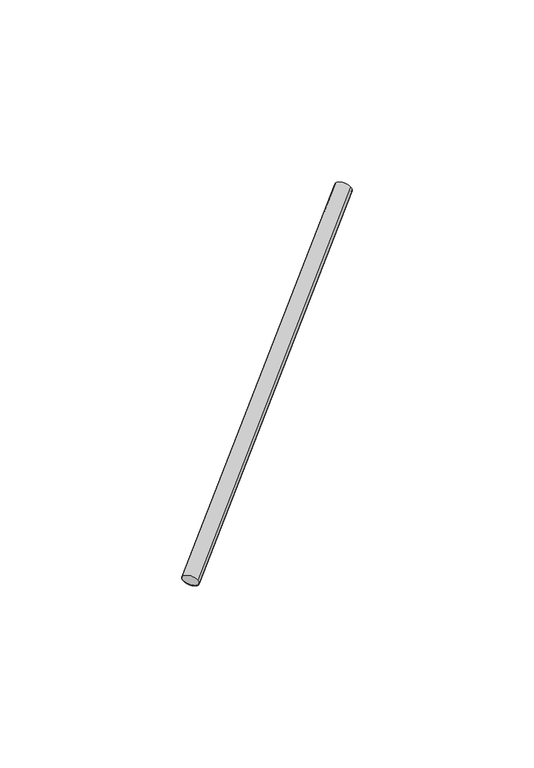
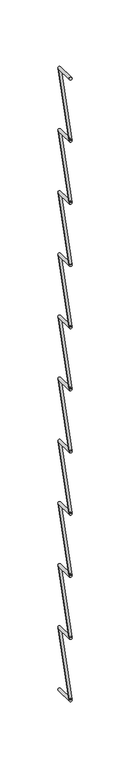
"""IFC4 building model written with IfcOpenShell, lengths in millimetres: proxy geometry, Pre-fab. (Vigota 7 - Pano 3)."""

from ifc_helpers import new_model, si_unit, point, frame, origin, origin_2d, place, context, project, spatial, circle_curve, trimmed, segment, composite_curve, outline, extrude, source, transform, mapped, element, save


def structural_framing_6d4e4e1a(model_context):
    return source(origin(), model_context, "Body", "SweptSolid", [
        extrude(outline(composite_curve([segment(trimmed(circle_curve(origin_2d(), 2.5), [point((2.5, 0.0))], [point((-2.5, 0.0))], False, "CARTESIAN"), True, "CONTINUOUS"), segment(trimmed(circle_curve(origin_2d(), 2.5), [point((-2.5, 0.0))], [point((2.5, 0.0))], False, "CARTESIAN"), True, "CONTINUOUS")], self_intersect=False)), frame((-42.0, 108.0, 1769.500535), z_axis=(-0.3218603428886276, -0.8276408817707567, 0.4598004898837537), x_axis=(0.8192319205108605, 3.936835275445103e-11, 0.5734623443750141)), (0.0, 0.0, 1.0), 130.491379),
        extrude(outline(composite_curve([segment(trimmed(circle_curve(origin_2d(), 2.5), [point((2.5, 0.0))], [point((-2.5, 0.0))], False, "CARTESIAN"), True, "CONTINUOUS"), segment(trimmed(circle_curve(origin_2d(), 2.5), [point((-2.5, 0.0))], [point((2.5, 0.0))], False, "CARTESIAN"), True, "CONTINUOUS")], self_intersect=False)), frame((-84.0, 0.0, 1829.500535), z_axis=(0.3218603428886276, 0.8276408817707567, 0.4598004898837537), x_axis=(0.8192319205108605, 3.936835275445103e-11, -0.5734623443750141)), (0.0, 0.0, 1.0), 130.491379),
        extrude(outline(composite_curve([segment(trimmed(circle_curve(origin_2d(), 2.5), [point((2.5, 0.0))], [point((-2.5, 0.0))], False, "CARTESIAN"), True, "CONTINUOUS"), segment(trimmed(circle_curve(origin_2d(), 2.5), [point((-2.5, 0.0))], [point((2.5, 0.0))], False, "CARTESIAN"), True, "CONTINUOUS")], self_intersect=False)), frame((-42.0, 108.0, 1889.500535), z_axis=(-0.3218603428886276, -0.8276408817707567, 0.4598004898837537), x_axis=(0.8192319205108605, 3.936835275445103e-11, 0.5734623443750141)), (0.0, 0.0, 1.0), 130.491379),
        extrude(outline(composite_curve([segment(trimmed(circle_curve(origin_2d(), 2.5), [point((2.5, 0.0))], [point((-2.5, 0.0))], False, "CARTESIAN"), True, "CONTINUOUS"), segment(trimmed(circle_curve(origin_2d(), 2.5), [point((-2.5, 0.0))], [point((2.5, 0.0))], False, "CARTESIAN"), True, "CONTINUOUS")], self_intersect=False)), frame((-84.0, 0.0, 1949.500535), z_axis=(0.3218603428886276, 0.8276408817707567, 0.4598004898837537), x_axis=(0.8192319205108605, 3.936835275445103e-11, -0.5734623443750141)), (0.0, 0.0, 1.0), 130.491379),
        extrude(outline(composite_curve([segment(trimmed(circle_curve(origin_2d(), 2.5), [point((2.5, 0.0))], [point((-2.5, 0.0))], False, "CARTESIAN"), True, "CONTINUOUS"), segment(trimmed(circle_curve(origin_2d(), 2.5), [point((-2.5, 0.0))], [point((2.5, 0.0))], False, "CARTESIAN"), True, "CONTINUOUS")], self_intersect=False)), frame((-42.0, 108.0, 2009.500535), z_axis=(-0.3218603428886276, -0.8276408817707567, 0.4598004898837537), x_axis=(0.8192319205108605, 3.936835275445103e-11, 0.5734623443750141)), (0.0, 0.0, 1.0), 130.491379),
        extrude(outline(composite_curve([segment(trimmed(circle_curve(origin_2d(), 2.5), [point((2.5, 0.0))], [point((-2.5, 0.0))], False, "CARTESIAN"), True, "CONTINUOUS"), segment(trimmed(circle_curve(origin_2d(), 2.5), [point((-2.5, 0.0))], [point((2.5, 0.0))], False, "CARTESIAN"), True, "CONTINUOUS")], self_intersect=False)), frame((-84.0, 0.0, 2069.500535), z_axis=(0.3218603428886276, 0.8276408817707567, 0.4598004898837537), x_axis=(0.8192319205108605, 3.936835275445103e-11, -0.5734623443750141)), (0.0, 0.0, 1.0), 130.491379),
        extrude(outline(composite_curve([segment(trimmed(circle_curve(origin_2d(), 2.5), [point((2.5, 0.0))], [point((-2.5, 0.0))], False, "CARTESIAN"), True, "CONTINUOUS"), segment(trimmed(circle_curve(origin_2d(), 2.5), [point((-2.5, 0.0))], [point((2.5, 0.0))], False, "CARTESIAN"), True, "CONTINUOUS")], self_intersect=False)), frame((-42.0, 108.0, 2129.500535), z_axis=(-0.3218603428886276, -0.8276408817707567, 0.4598004898837537), x_axis=(0.8192319205108605, 3.936835275445103e-11, 0.5734623443750141)), (0.0, 0.0, 1.0), 130.491379),
        extrude(outline(composite_curve([segment(trimmed(circle_curve(origin_2d(), 2.5), [point((2.5, 0.0))], [point((-2.5, 0.0))], False, "CARTESIAN"), True, "CONTINUOUS"), segment(trimmed(circle_curve(origin_2d(), 2.5), [point((-2.5, 0.0))], [point((2.5, 0.0))], False, "CARTESIAN"), True, "CONTINUOUS")], self_intersect=False)), frame((-84.0, 0.0, 2189.500535), z_axis=(0.3218603428886276, 0.8276408817707567, 0.4598004898837537), x_axis=(0.8192319205108605, 3.936835275445103e-11, -0.5734623443750141)), (0.0, 0.0, 1.0), 130.491379),
        extrude(outline(composite_curve([segment(trimmed(circle_curve(origin_2d(), 2.5), [point((2.5, 0.0))], [point((-2.5, 0.0))], False, "CARTESIAN"), True, "CONTINUOUS"), segment(trimmed(circle_curve(origin_2d(), 2.5), [point((-2.5, 0.0))], [point((2.5, 0.0))], False, "CARTESIAN"), True, "CONTINUOUS")], self_intersect=False)), frame((-42.0, 108.0, 2249.500535), z_axis=(-0.3218603428886276, -0.8276408817707567, 0.4598004898837537), x_axis=(0.8192319205108605, 3.936835275445103e-11, 0.5734623443750141)), (0.0, 0.0, 1.0), 130.491379),
        extrude(outline(composite_curve([segment(trimmed(circle_curve(origin_2d(), 2.5), [point((2.5, 0.0))], [point((-2.5, 0.0))], False, "CARTESIAN"), True, "CONTINUOUS"), segment(trimmed(circle_curve(origin_2d(), 2.5), [point((-2.5, 0.0))], [point((2.5, 0.0))], False, "CARTESIAN"), True, "CONTINUOUS")], self_intersect=False)), frame((-84.0, 0.0, 2309.500535), z_axis=(0.3218603428886276, 0.8276408817707567, 0.4598004898837537), x_axis=(0.8192319205108605, 3.936835275445103e-11, -0.5734623443750141)), (0.0, 0.0, 1.0), 130.491379),
        extrude(outline(composite_curve([segment(trimmed(circle_curve(origin_2d(), 2.5), [point((2.5, 0.0))], [point((-2.5, 0.0))], False, "CARTESIAN"), True, "CONTINUOUS"), segment(trimmed(circle_curve(origin_2d(), 2.5), [point((-2.5, 0.0))], [point((2.5, 0.0))], False, "CARTESIAN"), True, "CONTINUOUS")], self_intersect=False)), frame((-42.0, 108.0, 2369.500535), z_axis=(-0.3218603428886276, -0.8276408817707567, 0.4598004898837537), x_axis=(0.8192319205108605, 3.936835275445103e-11, 0.5734623443750141)), (0.0, 0.0, 1.0), 130.491379),
        extrude(outline(composite_curve([segment(trimmed(circle_curve(origin_2d(), 2.5), [point((2.5, 0.0))], [point((-2.5, 0.0))], False, "CARTESIAN"), True, "CONTINUOUS"), segment(trimmed(circle_curve(origin_2d(), 2.5), [point((-2.5, 0.0))], [point((2.5, 0.0))], False, "CARTESIAN"), True, "CONTINUOUS")], self_intersect=False)), frame((-84.0, 0.0, 2429.500535), z_axis=(0.3218603428886276, 0.8276408817707567, 0.4598004898837537), x_axis=(0.8192319205108605, 3.936835275445103e-11, -0.5734623443750141)), (0.0, 0.0, 1.0), 130.491379),
        extrude(outline(composite_curve([segment(trimmed(circle_curve(origin_2d(), 2.5), [point((2.5, 0.0))], [point((-2.5, 0.0))], False, "CARTESIAN"), True, "CONTINUOUS"), segment(trimmed(circle_curve(origin_2d(), 2.5), [point((-2.5, 0.0))], [point((2.5, 0.0))], False, "CARTESIAN"), True, "CONTINUOUS")], self_intersect=False)), frame((-42.0, 108.0, 2489.500535), z_axis=(-0.3218603428886276, -0.8276408817707567, 0.4598004898837537), x_axis=(0.8192319205108605, 3.936835275445103e-11, 0.5734623443750141)), (0.0, 0.0, 1.0), 130.491379),
        extrude(outline(composite_curve([segment(trimmed(circle_curve(origin_2d(), 2.5), [point((2.5, 0.0))], [point((-2.5, 0.0))], False, "CARTESIAN"), True, "CONTINUOUS"), segment(trimmed(circle_curve(origin_2d(), 2.5), [point((-2.5, 0.0))], [point((2.5, 0.0))], False, "CARTESIAN"), True, "CONTINUOUS")], self_intersect=False)), frame((-84.0, 0.0, 2549.500535), z_axis=(0.3218603428886276, 0.8276408817707567, 0.4598004898837537), x_axis=(0.8192319205108605, 3.936835275445103e-11, -0.5734623443750141)), (0.0, 0.0, 1.0), 130.491379),
        extrude(outline(composite_curve([segment(trimmed(circle_curve(origin_2d(), 2.5), [point((2.5, 0.0))], [point((-2.5, 0.0))], False, "CARTESIAN"), True, "CONTINUOUS"), segment(trimmed(circle_curve(origin_2d(), 2.5), [point((-2.5, 0.0))], [point((2.5, 0.0))], False, "CARTESIAN"), True, "CONTINUOUS")], self_intersect=False)), frame((-42.0, 108.0, 2609.500535), z_axis=(-0.3218603428886276, -0.8276408817707567, 0.4598004898837537), x_axis=(0.8192319205108605, 3.936835275445103e-11, 0.5734623443750141)), (0.0, 0.0, 1.0), 130.491379),
        extrude(outline(composite_curve([segment(trimmed(circle_curve(origin_2d(), 2.5), [point((2.5, 0.0))], [point((-2.5, 0.0))], False, "CARTESIAN"), True, "CONTINUOUS"), segment(trimmed(circle_curve(origin_2d(), 2.5), [point((-2.5, 0.0))], [point((2.5, 0.0))], False, "CARTESIAN"), True, "CONTINUOUS")], self_intersect=False)), frame((-84.0, 0.0, 2669.500535), z_axis=(0.3218603428886276, 0.8276408817707567, 0.4598004898837537), x_axis=(0.8192319205108605, 3.936835275445103e-11, -0.5734623443750141)), (0.0, 0.0, 1.0), 130.491379),
        extrude(outline(composite_curve([segment(trimmed(circle_curve(origin_2d(), 2.5), [point((2.5, 0.0))], [point((-2.5, 0.0))], False, "CARTESIAN"), True, "CONTINUOUS"), segment(trimmed(circle_curve(origin_2d(), 2.5), [point((-2.5, 0.0))], [point((2.5, 0.0))], False, "CARTESIAN"), True, "CONTINUOUS")], self_intersect=False)), frame((-42.0, 108.0, 2729.500535), z_axis=(-0.3218603428886276, -0.8276408817707567, 0.4598004898837537), x_axis=(0.8192319205108605, 3.936835275445103e-11, 0.5734623443750141)), (0.0, 0.0, 1.0), 130.491379),
        extrude(outline(composite_curve([segment(trimmed(circle_curve(origin_2d(), 2.5), [point((2.5, 0.0))], [point((-2.5, 0.0))], False, "CARTESIAN"), True, "CONTINUOUS"), segment(trimmed(circle_curve(origin_2d(), 2.5), [point((-2.5, 0.0))], [point((2.5, 0.0))], False, "CARTESIAN"), True, "CONTINUOUS")], self_intersect=False)), frame((-84.0, 0.0, 2789.500535), z_axis=(0.3218603428886276, 0.8276408817707567, 0.4598004898837537), x_axis=(0.8192319205108605, 3.936835275445103e-11, -0.5734623443750141)), (0.0, 0.0, 1.0), 130.491379),
        extrude(outline(composite_curve([segment(trimmed(circle_curve(origin_2d(), 2.5), [point((2.5, 0.0))], [point((-2.5, 0.0))], False, "CARTESIAN"), True, "CONTINUOUS"), segment(trimmed(circle_curve(origin_2d(), 2.5), [point((-2.5, 0.0))], [point((2.5, 0.0))], False, "CARTESIAN"), True, "CONTINUOUS")], self_intersect=False)), frame((-42.0, 108.0, 2849.500535), z_axis=(-0.3218603428886276, -0.8276408817707567, 0.4598004898837537), x_axis=(0.8192319205108605, 3.936835275445103e-11, 0.5734623443750141)), (0.0, 0.0, 1.0), 130.491379),
        extrude(outline(composite_curve([segment(trimmed(circle_curve(origin_2d(), 2.5), [point((2.5, 0.0))], [point((-2.5, 0.0))], False, "CARTESIAN"), True, "CONTINUOUS"), segment(trimmed(circle_curve(origin_2d(), 2.5), [point((-2.5, 0.0))], [point((2.5, 0.0))], False, "CARTESIAN"), True, "CONTINUOUS")], self_intersect=False)), frame((-84.0, 0.0, 2909.500535), z_axis=(0.3218603428886276, 0.8276408817707567, 0.4598004898837537), x_axis=(0.8192319205108605, 3.936835275445103e-11, -0.5734623443750141)), (0.0, 0.0, 1.0), 130.491379),
        extrude(outline(composite_curve([segment(trimmed(circle_curve(origin_2d(), 2.5), [point((2.5, 0.0))], [point((-2.5, 0.0))], False, "CARTESIAN"), True, "CONTINUOUS"), segment(trimmed(circle_curve(origin_2d(), 2.5), [point((-2.5, 0.0))], [point((2.5, 0.0))], False, "CARTESIAN"), True, "CONTINUOUS")], self_intersect=False)), frame((-42.0, 108.0, 2969.500535), z_axis=(-0.3218603428886276, -0.8276408817707567, 0.4598004898837537), x_axis=(0.8192319205108605, 3.936835275445103e-11, 0.5734623443750141)), (0.0, 0.0, 1.0), 130.491379),
    ])


if __name__ == "__main__":
    model = new_model("IFC4")
    model_context = context("Model", 3, world=origin())
    ifc_project = project(units=[si_unit("LENGTHUNIT", "METRE", prefix="MILLI")], contexts=[model_context])
    site = spatial("IfcSite", under=ifc_project)
    building = spatial("IfcBuilding", under=site)
    placement = place(None, origin())
    structural_framing_shape = structural_framing_6d4e4e1a(model_context)
    element("IfcBuildingElementProxy", 1, Name="Pre-fab. (Vigota 7 - Pano 3)", ObjectType="Pre-fab. (Vigota 7 - Pano 3)", at=placement, inside=building, context=model_context, shape_type="MappedRepresentation", body=[
        mapped(structural_framing_shape, transform((0.0, 0.0, 0.0), x_axis=(1.0, 0.0, 0.0), y_axis=(0.0, 1.0, 0.0), z_axis=(0.0, 0.0, 1.0))),
    ])
    save(model, "model.ifc")

# Revit data of these elements
# Element 1 (IfcBuildingElementProxy, "Pre-fab. (Vigota 7 - Pano 3)")
#   Materials on its faces: "Aço"
# Materials
#   "Aço": class "Metal", colour RGB 120 120 120, transparency 0, Description = "Aço estrutural A36 grau, ASTM B, acabamento laminado", Cost = 0
